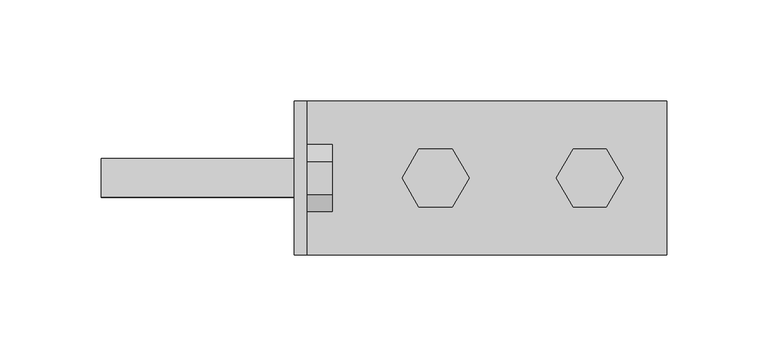
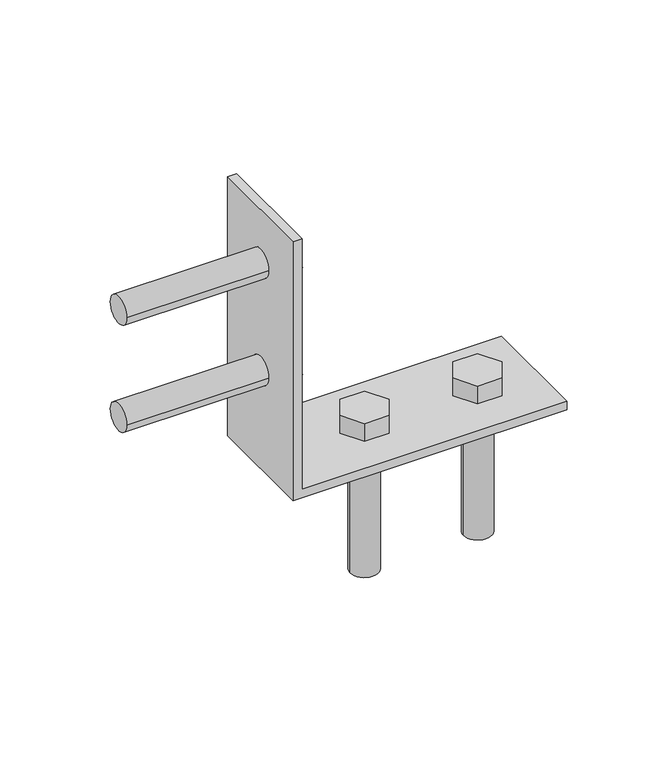
"""IFC4 building model written with IfcOpenShell, lengths in millimetres: fastener geometry, SIMPSON - HLPC/HLGPC Heavy Angles and Gussets : SIMPSON -HL73 - 3 X 7.25 - .75 Bolt - HDG."""

import ifcopenshell
import ifcopenshell.guid

model = None  # the IFC model being written
_history = None  # IfcOwnerHistory: only IFC2X3 demands one
_inside = {}  # id of a spatial element -> (the spatial element, [elements in it])
_under = {}  # id of a project, library or spatial element -> (it, [spatial elements below it])
_declared = {}  # id of a project -> (the project, [libraries it declares])
_typed = {}  # id of a type object -> (the type object, [elements of that type])
_made_of = {}  # id of a material, layer set ... -> (it, [elements and type objects made of it])


def new_model(schema):
    """Start an empty IFC model of exactly this schema.

    Asked for "IFC4X3", IfcOpenShell would pick the latest addendum, in which some entities
    have other attributes; the version numbers below select the first issue.
    IFC2X3 requires an IfcOwnerHistory on every rooted entity: one is made here for all.
    """
    global model, _history
    if schema == "IFC4X3":
        model = ifcopenshell.file(schema_version=(4, 3, 0, 0))
    else:
        model = ifcopenshell.file(schema=schema)
    _inside.clear()
    _under.clear()
    _declared.clear()
    _typed.clear()
    _made_of.clear()
    _history = None
    if model.schema == "IFC2X3":
        org = make("IfcOrganization", Name="unknown")
        user = make(
            "IfcPersonAndOrganization",
            ThePerson=make("IfcPerson", FamilyName="unknown"),
            TheOrganization=org,
        )
        app = make(
            "IfcApplication",
            ApplicationDeveloper=org,
            Version="unknown",
            ApplicationFullName="unknown",
            ApplicationIdentifier="unknown",
        )
        _history = make(
            "IfcOwnerHistory",
            OwningUser=user,
            OwningApplication=app,
            ChangeAction="ADDED",
            CreationDate=0,
        )
    return model


def make(cls, **values):
    """One entity of the class cls with the attributes given. An attribute that is None is left unset."""
    return model.create_entity(
        cls, **{name: value for name, value in values.items() if value is not None}
    )


def rooted(cls, **values):
    """An entity with a GlobalId (a new one), such as an element, a storey or a relation."""
    return make(cls, GlobalId=ifcopenshell.guid.new(), OwnerHistory=_history, **values)


def si_unit(unit_type, name, prefix=None):
    """IfcSIUnit, for example si_unit("LENGTHUNIT", "METRE", prefix="MILLI")."""
    return make("IfcSIUnit", UnitType=unit_type, Prefix=prefix, Name=name)


def assignment(units):
    """IfcUnitAssignment: the units of a project."""
    return None if units is None else make("IfcUnitAssignment", Units=units)


def point(xyz):
    """IfcCartesianPoint."""
    return None if xyz is None else make("IfcCartesianPoint", Coordinates=xyz)


def direction(xyz):
    """IfcDirection."""
    return None if xyz is None else make("IfcDirection", DirectionRatios=xyz)


def frame(location, z_axis=None, x_axis=None):
    """IfcAxis2Placement3D, a coordinate frame: its origin and axes. An axis left out is left unset."""
    return make(
        "IfcAxis2Placement3D",
        Location=point(location),
        Axis=direction(z_axis),
        RefDirection=direction(x_axis),
    )


def frame_2d(location, x_axis=None):
    """IfcAxis2Placement2D, a coordinate frame in the plane: its origin and x axis."""
    return make(
        "IfcAxis2Placement2D", Location=point(location), RefDirection=direction(x_axis)
    )


def origin():
    """The frame at (0, 0, 0) with its axes left unset."""
    return frame((0.0, 0.0, 0.0))


def place(relative_to, where):
    """IfcLocalPlacement: puts the frame where relative to a parent placement (None: the world)."""
    return make(
        "IfcLocalPlacement", PlacementRelTo=relative_to, RelativePlacement=where
    )


def context(
    kind, dimensions, precision=None, world=None, true_north=None, identifier=None
):
    """IfcGeometricRepresentationContext, for example the 3D "Model" context."""
    return make(
        "IfcGeometricRepresentationContext",
        ContextIdentifier=identifier,
        ContextType=kind,
        CoordinateSpaceDimension=dimensions,
        Precision=precision,
        WorldCoordinateSystem=world,
        TrueNorth=true_north,
    )


def project(units=None, contexts=None):
    """IfcProject with its units and contexts."""
    return rooted(
        "IfcProject",
        Name="project",
        RepresentationContexts=contexts,
        UnitsInContext=assignment(units),
    )


def spatial(cls, under=None, at=None, **own):
    """A site, building, storey or space (cls), placed at a placement, below another one or the project."""
    s = rooted(cls, ObjectPlacement=at, **own)
    if under is not None:
        _under.setdefault(under.id(), (under, []))[1].append(s)
    return s


def polyline(points):
    """IfcPolyline through the points."""
    return make("IfcPolyline", Points=[point(p) for p in points])


def circle_curve(where, radius):
    """IfcCircle in the frame where."""
    return make("IfcCircle", Position=where, Radius=radius)


def trimmed(basis, trim1, trim2, sense, master):
    """IfcTrimmedCurve: the piece of a basis curve between two trims."""
    return make(
        "IfcTrimmedCurve",
        BasisCurve=basis,
        Trim1=trim1,
        Trim2=trim2,
        SenseAgreement=sense,
        MasterRepresentation=master,
    )


def segment(curve, same_sense, transition):
    """IfcCompositeCurveSegment."""
    return make(
        "IfcCompositeCurveSegment",
        Transition=transition,
        SameSense=same_sense,
        ParentCurve=curve,
    )


def composite_curve(segments, self_intersect=None):
    """IfcCompositeCurve: segments joined end to end."""
    return make("IfcCompositeCurve", Segments=segments, SelfIntersect=self_intersect)


def outline(outer, holes=None, kind="AREA"):
    """IfcArbitraryClosedProfileDef: a profile drawn as a closed curve; with holes, ...WithVoids."""
    if holes is None:
        return make("IfcArbitraryClosedProfileDef", ProfileType=kind, OuterCurve=outer)
    return make(
        "IfcArbitraryProfileDefWithVoids",
        ProfileType=kind,
        OuterCurve=outer,
        InnerCurves=holes,
    )


def extrude(swept, where, along, depth):
    """IfcExtrudedAreaSolid: the profile swept, set in the frame where, extruded along a direction by depth."""
    return make(
        "IfcExtrudedAreaSolid",
        SweptArea=swept,
        Position=where,
        ExtrudedDirection=direction(along),
        Depth=depth,
    )


def shape(context_of_items, identifier, shape_type, items):
    """IfcShapeRepresentation: the items that make up one representation, for example the "Body"."""
    return make(
        "IfcShapeRepresentation",
        ContextOfItems=context_of_items,
        RepresentationIdentifier=identifier,
        RepresentationType=shape_type,
        Items=items,
    )


def source(mapping_origin, context_of_items, identifier, shape_type, items):
    """IfcRepresentationMap: a shape defined once, which mapped items show again and again."""
    return make(
        "IfcRepresentationMap",
        MappingOrigin=mapping_origin,
        MappedRepresentation=shape(context_of_items, identifier, shape_type, items),
    )


def transform(
    local_origin,
    x_axis=None,
    y_axis=None,
    z_axis=None,
    scale=None,
    scale2=None,
    scale3=None,
    uniform=True,
):
    """IfcCartesianTransformationOperator3D, or its non-uniform kind. x_axis, y_axis, z_axis: its Axis1, 2, 3."""
    if uniform:
        return make(
            "IfcCartesianTransformationOperator3D",
            Axis1=direction(x_axis),
            Axis2=direction(y_axis),
            LocalOrigin=point(local_origin),
            Scale=scale,
            Axis3=direction(z_axis),
        )
    return make(
        "IfcCartesianTransformationOperator3DnonUniform",
        Axis1=direction(x_axis),
        Axis2=direction(y_axis),
        LocalOrigin=point(local_origin),
        Scale=scale,
        Axis3=direction(z_axis),
        Scale2=scale2,
        Scale3=scale3,
    )


def mapped(mapping_source, mapping_target):
    """IfcMappedItem: shows the shape of a source again, moved by a transform."""
    return make(
        "IfcMappedItem", MappingSource=mapping_source, MappingTarget=mapping_target
    )


def made_of(thing, what):
    """Note that an element or type object is made of a material, layer set ...; save() writes the relation."""
    if what is not None:
        _made_of.setdefault(what.id(), (what, []))[1].append(thing)
    return thing


def element(
    cls,
    number,
    at=None,
    inside=None,
    cuts=None,
    type_object=None,
    material=None,
    context=None,
    identifier="Body",
    shape_type=None,
    held_by="IfcProductDefinitionShape",
    body=None,
    shapes=None,
    **own,
):
    """One element of the class cls, such as IfcWall. Its Tag is "e" and its number.

    at: its placement. inside: the storey or other place that contains it. cuts: it is an
    opening in that element (IfcRelVoidsElement). A single representation is given by context,
    identifier, shape_type and body (its items); several are given by shapes. held_by: the class
    of the entity that holds the representations. save() writes the other relations.
    """
    e = rooted(cls, Tag="e%d" % number, ObjectPlacement=at, **own)
    if body is not None:
        shapes = [shape(context, identifier, shape_type, body)]
    if shapes is not None:
        e.Representation = make(held_by, Representations=shapes)
    if inside is not None:
        _inside.setdefault(inside.id(), (inside, []))[1].append(e)
    if cuts is not None:
        rooted(
            "IfcRelVoidsElement", RelatingBuildingElement=cuts, RelatedOpeningElement=e
        )
    if type_object is not None:
        _typed.setdefault(type_object.id(), (type_object, []))[1].append(e)
    return made_of(e, material)


def aggregate(whole, parts):
    """IfcRelAggregates: a whole, such as a stair, and the parts it consists of."""
    return rooted("IfcRelAggregates", RelatingObject=whole, RelatedObjects=parts)


def save(model, path):
    """Write the relations noted so far, then the file.

    IfcRelAggregates (storeys below a building ...), IfcRelContainedInSpatialStructure (elements
    in a storey), IfcRelDefinesByType, IfcRelAssociatesMaterial and IfcRelDeclares: one each for
    every whole, place, type object, material and project.
    """
    for whole, parts in _under.values():
        aggregate(whole, parts)
    for where, things in _inside.values():
        rooted(
            "IfcRelContainedInSpatialStructure",
            RelatedElements=things,
            RelatingStructure=where,
        )
    for kind, things in _typed.values():
        rooted("IfcRelDefinesByType", RelatedObjects=things, RelatingType=kind)
    for what, things in _made_of.values():
        rooted("IfcRelAssociatesMaterial", RelatedObjects=things, RelatingMaterial=what)
    for by, libraries in _declared.values():
        rooted("IfcRelDeclares", RelatingContext=by, RelatedDefinitions=libraries)
    model.write(path)


def plane_surface(at):
    """IfcPlane: the flat surface through the origin of the frame at, square to its z axis."""
    return make("IfcPlane", Position=at)


def revolved_surface(curve, axis_point, axis_direction):
    """IfcSurfaceOfRevolution: the curve turned about the line through axis_point along axis_direction."""
    return make(
        "IfcSurfaceOfRevolution",
        SweptCurve=make("IfcArbitraryOpenProfileDef", ProfileType="CURVE", Curve=curve),
        AxisPosition=make("IfcAxis1Placement", Location=point(axis_point), Axis=direction(axis_direction)),
    )


def advanced_brep(points, edges, surfaces, faces):
    """IfcAdvancedBrep: a solid bounded by faces that lie on surfaces and meet in shared edges.

    An edge is (start, end): straight between two places in points (the first is 0);
    or (start, end, curve); or (start, end, curve, False) where it runs against its curve.
    A face is (place in surfaces, loops), or (place, loops, False) where it looks against
    its surface's normal. A loop lists edges by number (the first is 1), with a minus sign
    where the edge is run from its end to its start. The first loop is the outer one.
    """
    corners = [point(p) for p in points]
    vertices = [make("IfcVertexPoint", VertexGeometry=c) for c in corners]
    made = []
    for start, end, *more in edges:
        made.append(
            make(
                "IfcEdgeCurve",
                EdgeStart=vertices[start],
                EdgeEnd=vertices[end],
                EdgeGeometry=more[0] if more else make("IfcPolyline", Points=[corners[start], corners[end]]),
                SameSense=more[1] if len(more) > 1 else True,
            )
        )
    hull = []
    for where, loops, *sense in faces:
        bounds = []
        for j, loop in enumerate(loops):
            ring = [make("IfcOrientedEdge", EdgeElement=made[abs(k) - 1], Orientation=k > 0) for k in loop]
            bounds.append(
                make(
                    "IfcFaceOuterBound" if j == 0 else "IfcFaceBound",
                    Bound=make("IfcEdgeLoop", EdgeList=ring),
                    Orientation=True,
                )
            )
        hull.append(make("IfcAdvancedFace", Bounds=bounds, FaceSurface=surfaces[where], SameSense=sense[0] if sense else True))
    return make("IfcAdvancedBrep", Outer=make("IfcClosedShell", CfsFaces=hull))


def fastener_2b3ee341(model_context):
    return source(origin(), model_context, "Body", "SolidModel", [
        extrude(outline(composite_curve([segment(trimmed(circle_curve(frame_2d((0.0, 69.85)), 9.525), [point((-9.525, 69.85))], [point((9.525, 69.85))], False, "CARTESIAN"), True, "CONTINUOUS"), segment(trimmed(circle_curve(frame_2d((0.0, 69.85)), 9.525), [point((9.525, 69.85))], [point((-9.525, 69.85))], False, "CARTESIAN"), True, "CONTINUOUS")], self_intersect=False)), frame((-95.5476562, 0.0, 0.0), z_axis=(1.0, 0.0, 0.0), x_axis=(0.0, 1.0, 0.0)), (0.0, 0.0, 1.0), 101.6),
        extrude(outline(polyline([(-16.4977839, 69.85), (-8.248892, 84.1375), (8.248892, 84.1375), (16.4977839, 69.85), (8.248892, 55.5625), (-8.248892, 55.5625), (-16.4977839, 69.85)])), frame((6.0523438, 0.0, 0.0), z_axis=(1.0, 0.0, 0.0), x_axis=(0.0, 1.0, 0.0)), (0.0, 0.0, 1.0), 12.7),
        extrude(outline(composite_curve([segment(trimmed(circle_curve(frame_2d((0.0, 146.05)), 9.525), [point((-9.525, 146.05))], [point((9.525, 146.05))], False, "CARTESIAN"), True, "CONTINUOUS"), segment(trimmed(circle_curve(frame_2d((0.0, 146.05)), 9.525), [point((9.525, 146.05))], [point((-9.525, 146.05))], False, "CARTESIAN"), True, "CONTINUOUS")], self_intersect=False)), frame((-95.5476562, 0.0, 0.0), z_axis=(1.0, 0.0, 0.0), x_axis=(0.0, 1.0, 0.0)), (0.0, 0.0, 1.0), 101.6),
        extrude(outline(polyline([(-16.4977839, 146.05), (-8.248892, 160.3375), (8.248892, 160.3375), (16.4977839, 146.05), (8.248892, 131.7625), (-8.248892, 131.7625), (-16.4977839, 146.05)])), frame((6.0523438, 0.0, 0.0), z_axis=(1.0, 0.0, 0.0), x_axis=(0.0, 1.0, 0.0)), (0.0, 0.0, 1.0), 12.7),
        extrude(outline(composite_curve([segment(trimmed(circle_curve(frame_2d((146.05, 0.0)), 9.525), [point((136.525, 0.0))], [point((155.575, 0.0))], False, "CARTESIAN"), True, "CONTINUOUS"), segment(trimmed(circle_curve(frame_2d((146.05, 0.0)), 9.525), [point((155.575, 0.0))], [point((136.525, 0.0))], False, "CARTESIAN"), True, "CONTINUOUS")], self_intersect=False)), frame((0.0, 0.0, -95.5476563), z_axis=(0.0, 0.0, 1.0), x_axis=(1.0, 0.0, 0.0)), (0.0, 0.0, 1.0), 101.6),
        extrude(outline(polyline([(129.5522161, 0.0), (137.801108, 14.2875), (154.298892, 14.2875), (162.5477839, 0.0), (154.298892, -14.2875), (137.801108, -14.2875), (129.5522161, 0.0)])), frame((0.0, 0.0, 6.0523437), z_axis=(0.0, 0.0, 1.0), x_axis=(1.0, 0.0, 0.0)), (0.0, 0.0, 1.0), 12.7),
        extrude(outline(composite_curve([segment(trimmed(circle_curve(frame_2d((69.85, 0.0)), 9.525), [point((60.325, 0.0))], [point((79.375, 0.0))], False, "CARTESIAN"), True, "CONTINUOUS"), segment(trimmed(circle_curve(frame_2d((69.85, 0.0)), 9.525), [point((79.375, 0.0))], [point((60.325, 0.0))], False, "CARTESIAN"), True, "CONTINUOUS")], self_intersect=False)), frame((0.0, 0.0, -95.5476563), z_axis=(0.0, 0.0, 1.0), x_axis=(1.0, 0.0, 0.0)), (0.0, 0.0, 1.0), 101.6),
        extrude(outline(polyline([(53.3522161, 0.0), (61.601108, 14.2875), (78.098892, 14.2875), (86.3477839, 0.0), (78.098892, -14.2875), (61.601108, -14.2875), (53.3522161, 0.0)])), frame((0.0, 0.0, 6.0523437), z_axis=(0.0, 0.0, 1.0), x_axis=(1.0, 0.0, 0.0)), (0.0, 0.0, 1.0), 12.7),
        advanced_brep(
        [(6.0523438, 38.1, 184.15), (6.0523438, -38.1, 184.15), (6.0523438, -38.1, 6.0523437), (6.0523438, 38.1, 6.0523437), (6.0523438, 9.525, 69.85), (6.0523438, -9.525, 69.85), (6.0523438, 9.525, 146.05), (6.0523438, -9.525, 146.05), (0.0, -38.1, 184.15), (0.0, 38.1, 184.15), (0.0, 38.1, 0.0), (0.0, -38.1, 0.0), (0.0, -9.525, 69.85), (0.0, 9.525, 69.85), (0.0, -9.525, 146.05), (0.0, 9.525, 146.05), (184.15, -38.1, 0.0), (184.15, -38.1, 6.0523437), (184.15, 38.1, 6.0523437), (184.15, 38.1, 0.0), (79.375, 0.0, 6.0523437), (60.325, 0.0, 6.0523437), (155.575, 0.0, 6.0523437), (136.525, 0.0, 6.0523437), (60.325, 0.0, 0.0), (79.375, 0.0, 0.0), (136.525, 0.0, 0.0), (155.575, 0.0, 0.0)],
        [
            (0, 1),
            (1, 2),
            (2, 3),
            (3, 0),
            (4, 5, circle_curve(frame((6.0523438, 0.0, 69.85), z_axis=(-1.0, 0.0, 0.0), x_axis=(0.0, 1.0, 0.0)), 9.525)),
            (5, 4, circle_curve(frame((6.0523438, 0.0, 69.85), z_axis=(-1.0, 0.0, 0.0), x_axis=(0.0, 1.0, 0.0)), 9.525)),
            (6, 7, circle_curve(frame((6.0523438, 0.0, 146.05), z_axis=(-1.0, 0.0, 0.0), x_axis=(0.0, 1.0, 0.0)), 9.525)),
            (7, 6, circle_curve(frame((6.0523438, 0.0, 146.05), z_axis=(-1.0, 0.0, 0.0), x_axis=(0.0, 1.0, 0.0)), 9.525)),
            (8, 9),
            (9, 10),
            (10, 11),
            (11, 8),
            (12, 13, circle_curve(frame((0.0, 0.0, 69.85), z_axis=(1.0, 0.0, 0.0), x_axis=(0.0, 1.0, 0.0)), 9.525)),
            (13, 12, circle_curve(frame((0.0, 0.0, 69.85), z_axis=(1.0, 0.0, 0.0), x_axis=(0.0, 1.0, 0.0)), 9.525)),
            (14, 15, circle_curve(frame((0.0, 0.0, 146.05), z_axis=(1.0, 0.0, 0.0), x_axis=(0.0, 1.0, 0.0)), 9.525)),
            (15, 14, circle_curve(frame((0.0, 0.0, 146.05), z_axis=(1.0, 0.0, 0.0), x_axis=(0.0, 1.0, 0.0)), 9.525)),
            (0, 9),
            (8, 1),
            (11, 16),
            (16, 17),
            (17, 2),
            (3, 18),
            (18, 19),
            (19, 10),
            (17, 18),
            (20, 21, circle_curve(frame((69.85, 0.0, 6.0523437), z_axis=(0.0, 0.0, -1.0), x_axis=(1.0, 0.0, 0.0)), 9.525)),
            (21, 20, circle_curve(frame((69.85, 0.0, 6.0523437), z_axis=(0.0, 0.0, -1.0), x_axis=(1.0, 0.0, 0.0)), 9.525)),
            (22, 23, circle_curve(frame((146.05, 0.0, 6.0523437), z_axis=(0.0, 0.0, -1.0), x_axis=(1.0, 0.0, 0.0)), 9.525)),
            (23, 22, circle_curve(frame((146.05, 0.0, 6.0523437), z_axis=(0.0, 0.0, -1.0), x_axis=(1.0, 0.0, 0.0)), 9.525)),
            (19, 16),
            (24, 25, circle_curve(frame((69.85, 0.0, 0.0), z_axis=(0.0, 0.0, 1.0), x_axis=(1.0, 0.0, 0.0)), 9.525)),
            (25, 24, circle_curve(frame((69.85, 0.0, 0.0), z_axis=(0.0, 0.0, 1.0), x_axis=(1.0, 0.0, 0.0)), 9.525)),
            (26, 27, circle_curve(frame((146.05, 0.0, 0.0), z_axis=(0.0, 0.0, 1.0), x_axis=(1.0, 0.0, 0.0)), 9.525)),
            (27, 26, circle_curve(frame((146.05, 0.0, 0.0), z_axis=(0.0, 0.0, 1.0), x_axis=(1.0, 0.0, 0.0)), 9.525)),
            (20, 25),
            (24, 21),
            (22, 27),
            (26, 23),
            (4, 13),
            (12, 5),
            (6, 15),
            (14, 7),
        ],
        [
            plane_surface(frame((6.0523438, -38.1, 184.15), z_axis=(1.0, 0.0, 0.0), x_axis=(0.0, -1.0, 0.0))),
            plane_surface(frame((0.0, -38.1, 184.15), z_axis=(-1.0, 0.0, 0.0), x_axis=(0.0, 1.0, 0.0))),
            plane_surface(frame((6.0523438, 38.1, 184.15), z_axis=(0.0, 0.0, 1.0), x_axis=(-1.0, 0.0, 0.0))),
            plane_surface(frame((6.0523438, -38.1, 184.15), z_axis=(0.0, -1.0, 0.0), x_axis=(-1.0, 0.0, 0.0))),
            plane_surface(frame((6.0523438, 38.1, 6.0523437), z_axis=(0.0, 1.0, 0.0), x_axis=(-1.0, 0.0, 0.0))),
            plane_surface(frame((0.0, 38.1, 6.0523437), z_axis=(0.0, 0.0, 1.0), x_axis=(-1.0, 0.0, 0.0))),
            plane_surface(frame((0.0, 38.1, 0.0), z_axis=(0.0, 0.0, -1.0), x_axis=(1.0, 0.0, 0.0))),
            plane_surface(frame((184.15, -38.1, 6.0523437), z_axis=(1.0, 0.0, 0.0), x_axis=(0.0, 0.0, -1.0))),
            revolved_surface(polyline([(79.375, 0.0, 6.0523437), (79.375, 0.0, 0.0)]), (69.85, 0.0, 0.0), (0.0, 0.0, 1.0)),
            revolved_surface(polyline([(155.57500000000002, 0.0, 6.0523437), (155.57500000000002, 0.0, 0.0)]), (146.05, 0.0, 0.0), (0.0, 0.0, 1.0)),
            revolved_surface(polyline([(6.0523438, 9.525, 69.85), (0.0, 9.525, 69.85)]), (0.0, 0.0, 69.85), (1.0, 0.0, 0.0)),
            revolved_surface(polyline([(6.0523438, 9.525, 146.05), (0.0, 9.525, 146.05)]), (0.0, 0.0, 146.05), (1.0, 0.0, 0.0)),
        ],
        [
            (0, [[1, 2, 3, 4], [5, 6], [7, 8]]),
            (1, [[9, 10, 11, 12], [13, 14], [15, 16]]),
            (2, [[-1, 17, -9, 18]]),
            (3, [[-2, -18, -12, 19, 20, 21]]),
            (4, [[-4, 22, 23, 24, -10, -17]]),
            (5, [[25, -22, -3, -21], [26, 27], [28, 29]]),
            (6, [[30, -19, -11, -24], [31, 32], [33, 34]]),
            (7, [[-25, -20, -30, -23]]),
            (8, [[35, -31, 36, -26]]),
            (8, [[-35, -27, -36, -32]]),
            (9, [[37, -33, 38, -28]]),
            (9, [[-37, -29, -38, -34]]),
            (10, [[39, -13, 40, -5]]),
            (10, [[-39, -6, -40, -14]]),
            (11, [[41, -15, 42, -7]]),
            (11, [[-41, -8, -42, -16]]),
        ],
    ),
    ])


if __name__ == "__main__":
    model = new_model("IFC4")
    model_context = context("Model", 3, world=origin())
    ifc_project = project(units=[si_unit("LENGTHUNIT", "METRE", prefix="MILLI")], contexts=[model_context])
    site = spatial("IfcSite", under=ifc_project)
    building = spatial("IfcBuilding", under=site)
    placement = place(None, origin())
    fastener_shape = fastener_2b3ee341(model_context)
    element("IfcFastener", 1, ObjectType="SIMPSON - HLPC/HLGPC Heavy Angles and Gussets : SIMPSON -HL73 - 3 X 7.25 - .75 Bolt - HDG", at=placement, inside=building, context=model_context, shape_type="MappedRepresentation", body=[
        mapped(fastener_shape, transform((0.0, 0.0, 0.0), x_axis=(1.0, 0.0, 0.0), y_axis=(0.0, 1.0, 0.0), z_axis=(0.0, 0.0, 1.0))),
    ])
    save(model, "model.ifc")

# Revit data of these elements
# Type "SIMPSON - HLPC/HLGPC Heavy Angles and Gussets : SIMPSON -HL73 - 3 X 7.25 - .75 Bolt - HDG"
#   URL = "https://www.strongtie.com/classiccollection_architecturalproductsgroup/hlpc-hlgpc_productgroup_wcc/p/hlpc.hlgpc"
#   L = 0' - 3"
#   Hole Radius = 0' - 0 3/8"
#   D4 = 0' - 3"
#   D2 = 0' - 5"
#   D1 = 0' - 1 1/2"
#   D3 = 0' - 2 3/4"
#   Ga. = 0' - 0 61/256"
#   W1 & W2 = 0' - 7 1/4"
#   Default Elevation = 4' - 0"
#   Bolt Visibility - 3B = no
#   Bolt Visibility - 3A = no
#   Bolt Visibility - 2B = no
#   Bolt Visibility - 2A = no
#   Bolt Visibility - 1B = yes
#   Bolt Visibility - 1A = yes
#   Bolt Visibility = yes
#   Bolt Size = element 1298415
# Element 1 (IfcFastener, "SIMPSON - HLPC/HLGPC Heavy Angles and Gussets : SIMPSON -HL73 - 3 X 7.25 - .75 Bolt - HDG")
#   Materials on its faces: "1\" GALV. LAG BOLT (LENGTH = 1/2\" SHY OF GLULAM DEPTH) -  (GALV. THRU BOLT IF PLATE ON OPP. SIDE OF STRUCT MEMBER)"
# Materials
#   "1\" GALV. LAG BOLT (LENGTH = 1/2\" SHY OF GLULAM DEPTH) -  (GALV. THRU BOLT IF PLATE ON OPP. SIDE OF STRUCT MEMBER)": class "Generic", colour RGB 120 120 120, transparency 0, Cost = 0
